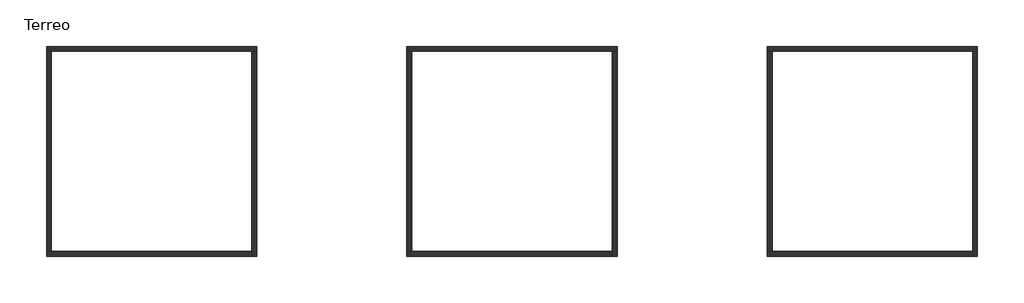
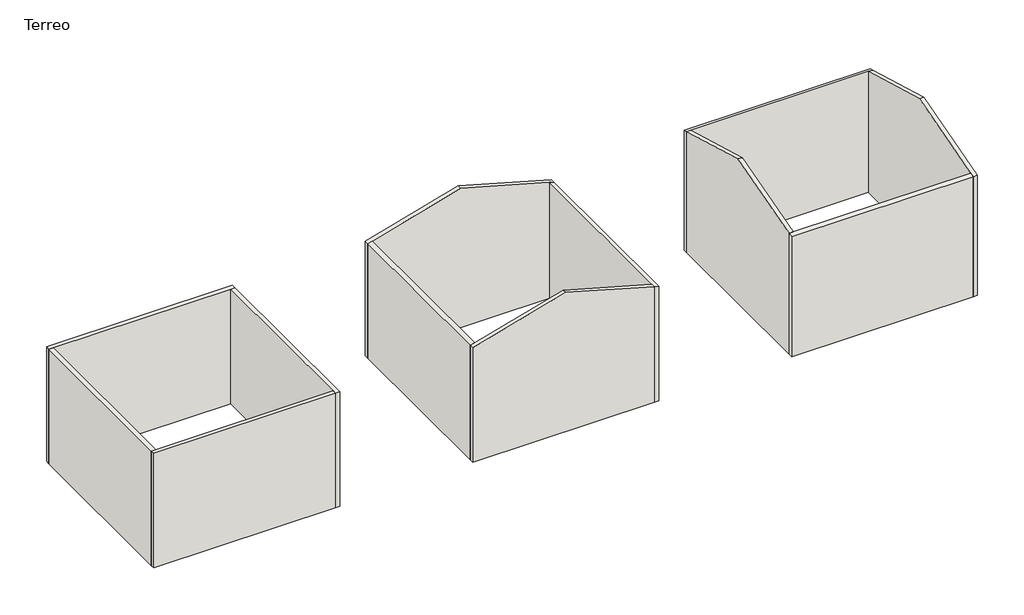
# One storey: 12 walls.
"""IFC4 building model written with IfcOpenShell, lengths in millimetres."""

from ifc_helpers import new_model, si_unit, frame, origin, origin_with_axes, place, context, project, spatial, polyline, outline, extrude, faceted_brep, element, save

model = new_model("IFC4")

# Units and contexts
model_context = context("Model", 3, world=origin())
ifc_project = project(units=[si_unit("LENGTHUNIT", "METRE", prefix="MILLI")], contexts=[model_context])

# Site, building, storey
site = spatial("IfcSite", under=ifc_project)
building = spatial("IfcBuilding", under=site)
storey = spatial("IfcBuildingStorey", under=building, Name="Terreo", Elevation=0.0)

# Walls
placement = place(None, origin())
element("IfcWall", 1, ObjectType="Parede Bloco 19 cm - Pintura / Pintura", at=placement, inside=storey, context=model_context, shape_type="Brep", body=[
    faceted_brep([(-5587.3421872, 4601.1974788, 0.0), (-5378.1421872, 4601.1974788, 0.0), (3412.6578128, 4601.1974788, 0.0), (3621.8578128, 4601.1974788, 0.0), (3621.8578128, 4601.1974788, 6000.0), (3412.6578128, 4601.1974788, 6000.0), (-5378.1421872, 4601.1974788, 6000.0), (-5587.3421872, 4601.1974788, 6000.0), (-5587.3421872, 4810.3974788, 0.0), (-5587.3421872, 4810.3974788, 6000.0), (3621.8578128, 4810.3974788, 6000.0), (3621.8578128, 4810.3974788, 0.0)], [[[0, 1, 2, 3, 4, 5, 6, 7]], [[8, 9, 10, 11]], [[3, 2, 1, 0, 8, 11]], [[7, 6, 5, 4, 10, 9]], [[4, 3, 11, 10]], [[0, 7, 9, 8]]]),
])
element("IfcWall", 2, ObjectType="Parede Bloco 19 cm - Pintura / Pintura", at=placement, inside=storey, context=model_context, shape_type="Brep", body=[
    faceted_brep([(3412.6578128, 4601.1974788, 0.0), (3412.6578128, -4189.6025212, 0.0), (3412.6578128, -4398.8025212, 0.0), (3412.6578128, -4398.8025212, 6000.0), (3412.6578128, -4189.6025212, 6000.0), (3412.6578128, 4601.1974788, 6000.0), (3621.8578128, 4601.1974788, 0.0), (3621.8578128, 4601.1974788, 6000.0), (3621.8578128, -4398.8025212, 6000.0), (3621.8578128, -4398.8025212, 0.0)], [[[0, 1, 2, 3, 4, 5]], [[6, 7, 8, 9]], [[2, 1, 0, 6, 9]], [[5, 4, 3, 8, 7]], [[0, 5, 7, 6]], [[3, 2, 9, 8]]]),
])
element("IfcWall", 3, ObjectType="Parede Bloco 19 cm - Pintura / Pintura", at=placement, inside=storey, context=model_context, shape_type="Brep", body=[
    faceted_brep([(3412.6578128, -4189.6025212, 0.0), (-5378.1421872, -4189.6025212, 0.0), (-5587.3421872, -4189.6025212, 0.0), (-5587.3421872, -4189.6025212, 6000.0), (-5378.1421872, -4189.6025212, 6000.0), (3412.6578128, -4189.6025212, 6000.0), (3412.6578128, -4398.8025212, 0.0), (3412.6578128, -4398.8025212, 6000.0), (-5587.3421872, -4398.8025212, 6000.0), (-5587.3421872, -4398.8025212, 0.0)], [[[0, 1, 2, 3, 4, 5]], [[6, 7, 8, 9]], [[2, 1, 0, 6, 9]], [[5, 4, 3, 8, 7]], [[0, 5, 7, 6]], [[3, 2, 9, 8]]]),
])
element("IfcWall", 4, ObjectType="Parede Bloco 19 cm - Pintura / Pintura", at=placement, inside=storey, context=model_context, shape_type="SweptSolid", body=[
    extrude(outline(polyline([(-5378.1421872, 4601.1974788), (-5378.1421872, -4189.6025212), (-5587.3421872, -4189.6025212), (-5587.3421872, 4601.1974788), (-5378.1421872, 4601.1974788)])), origin_with_axes(), (0.0, 0.0, 1.0), 6000.0),
])
element("IfcWall", 5, ObjectType="Parede Bloco 19 cm - Pintura / Pintura", at=placement, inside=storey, context=model_context, shape_type="Brep", body=[
    faceted_brep([(10212.6578128, 4601.1974788, 0.0), (10421.8578128, 4601.1974788, 0.0), (19212.6578128, 4601.1974788, 0.0), (19421.8578128, 4601.1974788, 0.0), (19421.8578128, 4601.1974788, 6000.0), (19212.6578128, 4601.1974788, 6058.576), (14817.2578128, 4601.1974788, 7289.288), (10421.8578128, 4601.1974788, 6058.576), (10212.6578128, 4601.1974788, 6000.0), (10212.6578128, 4810.3974788, 0.0), (10212.6578128, 4810.3974788, 6000.0), (14817.2578128, 4810.3974788, 7289.288), (19421.8578128, 4810.3974788, 6000.0), (19421.8578128, 4810.3974788, 0.0)], [[[0, 1, 2, 3, 4, 5, 6, 7, 8]], [[9, 10, 11, 12, 13]], [[3, 2, 1, 0, 9, 13]], [[4, 3, 13, 12]], [[0, 8, 10, 9]], [[8, 7, 6, 11, 10]], [[6, 5, 4, 12, 11]]]),
])
element("IfcWall", 6, ObjectType="Parede Bloco 19 cm - Pintura / Pintura", at=placement, inside=storey, context=model_context, shape_type="Brep", body=[
    faceted_brep([(19212.6578128, 4601.1974788, 0.0), (19212.6578128, -4189.6025212, 0.0), (19212.6578128, -4398.8025212, 0.0), (19212.6578128, -4398.8025212, 6058.576), (19212.6578128, -4189.6025212, 6058.576), (19212.6578128, 4601.1974788, 6058.576), (19421.8578128, 4601.1974788, 0.0), (19421.8578128, 4601.1974788, 6000.0), (19421.8578128, -4398.8025212, 6000.0), (19421.8578128, -4398.8025212, 0.0)], [[[0, 1, 2, 3, 4, 5]], [[6, 7, 8, 9]], [[2, 1, 0, 6, 9]], [[0, 5, 7, 6]], [[3, 2, 9, 8]], [[5, 4, 3, 8, 7]]]),
])
element("IfcWall", 7, ObjectType="Parede Bloco 19 cm - Pintura / Pintura", at=placement, inside=storey, context=model_context, shape_type="Brep", body=[
    faceted_brep([(19212.6578128, -4189.6025212, 0.0), (10421.8578128, -4189.6025212, 0.0), (10212.6578128, -4189.6025212, 0.0), (10212.6578128, -4189.6025212, 6000.0), (10421.8578128, -4189.6025212, 6058.576), (14817.2578128, -4189.6025212, 7289.288), (19212.6578128, -4189.6025212, 6058.576), (19212.6578128, -4398.8025212, 0.0), (19212.6578128, -4398.8025212, 6058.576), (14817.2578128, -4398.8025212, 7289.288), (10212.6578128, -4398.8025212, 6000.0), (10212.6578128, -4398.8025212, 0.0)], [[[0, 1, 2, 3, 4, 5, 6]], [[7, 8, 9, 10, 11]], [[2, 1, 0, 7, 11]], [[0, 6, 8, 7]], [[3, 2, 11, 10]], [[6, 5, 9, 8]], [[5, 4, 3, 10, 9]]]),
])
element("IfcWall", 8, ObjectType="Parede Bloco 19 cm - Pintura / Pintura", at=placement, inside=storey, context=model_context, shape_type="SweptSolid", body=[
    extrude(outline(polyline([(0.0, 10421.8578128), (6058.576, 10421.8578128), (6000.0, 10212.6578128), (0.0, 10212.6578128), (0.0, 10421.8578128)])), frame((0.0, -4189.6025212, 0.0), z_axis=(0.0, 1.0, 0.0), x_axis=(0.0, 0.0, 1.0)), (0.0, 0.0, 1.0), 8790.8),
])
element("IfcWall", 9, ObjectType="Parede Bloco 19 cm - Pintura / Pintura", at=placement, inside=storey, context=model_context, shape_type="Brep", body=[
    faceted_brep([(26012.6578128, 4601.1974788, 0.0), (26221.8578128, 4601.1974788, 0.0), (35012.6578128, 4601.1974788, 0.0), (35221.8578128, 4601.1974788, 0.0), (35221.8578128, 4601.1974788, 6338.576), (35012.6578128, 4601.1974788, 6338.576), (26221.8578128, 4601.1974788, 6338.576), (26012.6578128, 4601.1974788, 6338.576), (26012.6578128, 4810.3974788, 0.0), (26012.6578128, 4810.3974788, 6280.0), (35221.8578128, 4810.3974788, 6280.0), (35221.8578128, 4810.3974788, 0.0)], [[[0, 1, 2, 3, 4, 5, 6, 7]], [[8, 9, 10, 11]], [[3, 2, 1, 0, 8, 11]], [[4, 3, 11, 10]], [[0, 7, 9, 8]], [[7, 6, 5, 4, 10, 9]]]),
])
element("IfcWall", 10, ObjectType="Parede Bloco 19 cm - Pintura / Pintura", at=placement, inside=storey, context=model_context, shape_type="Brep", body=[
    faceted_brep([(35012.6578128, 4601.1974788, 0.0), (35012.6578128, -4189.6025212, 0.0), (35012.6578128, -4398.8025212, 0.0), (35012.6578128, -4398.8025212, 6280.0), (35012.6578128, -4189.6025212, 6338.576), (35012.6578128, 205.7974788, 7569.288), (35012.6578128, 4601.1974788, 6338.576), (35221.8578128, 4601.1974788, 0.0), (35221.8578128, 4601.1974788, 6338.576), (35221.8578128, 205.7974788, 7569.288), (35221.8578128, -4398.8025212, 6280.0), (35221.8578128, -4398.8025212, 0.0)], [[[0, 1, 2, 3, 4, 5, 6]], [[7, 8, 9, 10, 11]], [[2, 1, 0, 7, 11]], [[0, 6, 8, 7]], [[3, 2, 11, 10]], [[6, 5, 9, 8]], [[5, 4, 3, 10, 9]]]),
])
element("IfcWall", 11, ObjectType="Parede Bloco 19 cm - Pintura / Pintura", at=placement, inside=storey, context=model_context, shape_type="Brep", body=[
    faceted_brep([(35012.6578128, -4189.6025212, 0.0), (26221.8578128, -4189.6025212, 0.0), (26012.6578128, -4189.6025212, 0.0), (26012.6578128, -4189.6025212, 6338.576), (26221.8578128, -4189.6025212, 6338.576), (35012.6578128, -4189.6025212, 6338.576), (35012.6578128, -4398.8025212, 0.0), (35012.6578128, -4398.8025212, 6280.0), (26012.6578128, -4398.8025212, 6280.0), (26012.6578128, -4398.8025212, 0.0)], [[[0, 1, 2, 3, 4, 5]], [[6, 7, 8, 9]], [[2, 1, 0, 6, 9]], [[0, 5, 7, 6]], [[3, 2, 9, 8]], [[5, 4, 3, 8, 7]]]),
])
element("IfcWall", 12, ObjectType="Parede Bloco 19 cm - Pintura / Pintura", at=placement, inside=storey, context=model_context, shape_type="SweptSolid", body=[
    extrude(outline(polyline([(-4189.6025212, 0.0), (-4189.6025212, 6338.576), (205.7974788, 7569.288), (4601.1974788, 6338.576), (4601.1974788, 0.0), (-4189.6025212, 0.0)])), frame((26012.6578128, 0.0, 0.0), z_axis=(1.0, 0.0, 0.0), x_axis=(0.0, 1.0, 0.0)), (0.0, 0.0, 1.0), 209.2),
])

save(model, "model.ifc")

# Revit data of these elements
# Project information
#   Project Issue Date = "Data de emissão"
#   Project Status = "Status do projeto"
#   Client Name = "Proprietário"
#   Project Address = "Insira aqui o endereço"
#   Project Name = "Nome do projeto"
#   Project Number = "0001"
# Type "Parede Bloco 19 cm - Pintura / Pintura"
#   Layers, outside or top first: 0.0016 m "Pintura Látex PVA" (function 4); 0.008 m "Gesso" (function 4); 0.19 m "Alvenaria - Bloco de Cerâmico - 14cm" (function 1); 0.008 m "Gesso" (function 2); 0.0016 m "Pintura Látex PVA" (function 4)
# Elements 1, 2, 3, 5, 6, 9, 11 (IfcWall, "Parede Bloco 19 cm - Pintura / Pintura")
#   Top Offset = 0.00 m
#   Base Offset = 0.00 m
#   wall height = 6.00 m
#   Phase Created = Construção nova
#   Base Constraint = Terreo
#   Top Constraint = Cobertura
#   Materials on its faces: "Pintura Látex PVA", "Material pré-definido de parede"
# Elements 4, 7, 8, 10, 12 (IfcWall, "Parede Bloco 19 cm - Pintura / Pintura")
#   Top Offset = 0.00 m
#   Base Offset = 0.00 m
#   wall height = 6.00 m
#   Phase Created = Construção nova
#   Base Constraint = Terreo
#   Top Constraint = Cobertura
#   Materials on its faces: "Material pré-definido de parede", "Pintura Látex PVA"
# Materials
#   "Pintura Látex PVA": class "Pintura", colour RGB 244 244 244, transparency 0, Cost = 0
#   "Gesso": class "Gesso", colour RGB 244 244 244, transparency 0, Cost = 0
#   "Alvenaria - Bloco de Cerâmico - 14cm": class "Cerâmica", colour RGB 255 255 255, transparency 0, Cost = 0
#   "Material pré-definido de parede": class "Diversos", colour RGB 128 128 128, transparency 0
